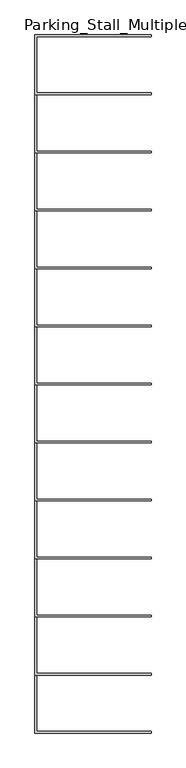
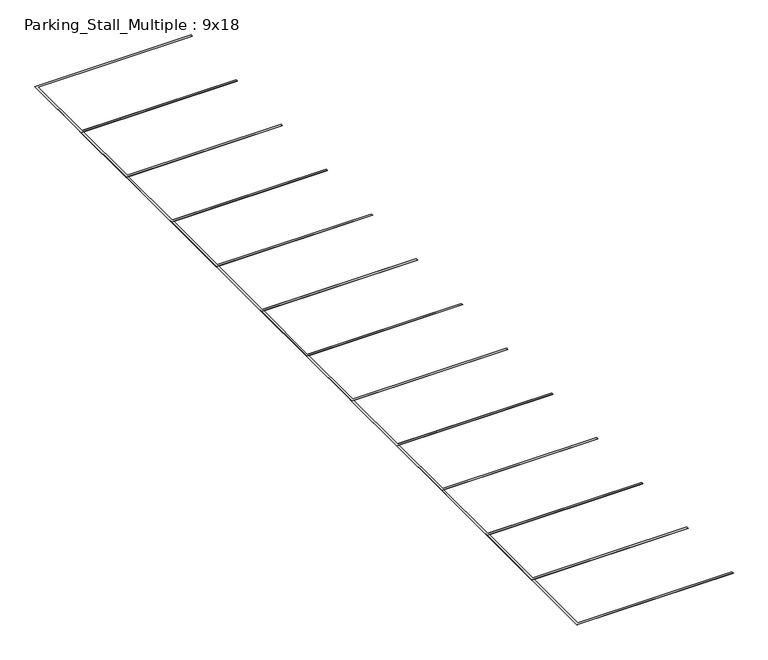
"""IFC4 building model written with IfcOpenShell, lengths in millimetres: proxy geometry, Parking_Stall_Multiple : 9x18."""

from ifc_helpers import new_model, si_unit, origin, origin_with_axes, place, context, project, spatial, polyline, outline, extrude, source, transform, mapped, element, save


def parking_stall_multiple_9x18_87ab82d0(model_context):
    return source(origin(), model_context, "Body", "SweptSolid", [
        extrude(outline(polyline([(5486.4, 30175.2), (0.0, 30175.2), (0.0, 32994.6), (5486.4, 32994.6), (5486.4, 32918.4), (76.2, 32918.4), (76.2, 30251.4), (5486.4, 30251.4), (5486.4, 30175.2)])), origin_with_axes(), (0.0, 0.0, 1.0), 6.35),
        extrude(outline(polyline([(5486.4, 27432.0), (0.0, 27432.0), (0.0, 30251.4), (5486.4, 30251.4), (5486.4, 30175.2), (76.2, 30175.2), (76.2, 27508.2), (5486.4, 27508.2), (5486.4, 27432.0)])), origin_with_axes(), (0.0, 0.0, 1.0), 6.35),
        extrude(outline(polyline([(5486.4, 24688.8), (0.0, 24688.8), (0.0, 27508.2), (5486.4, 27508.2), (5486.4, 27432.0), (76.2, 27432.0), (76.2, 24765.0), (5486.4, 24765.0), (5486.4, 24688.8)])), origin_with_axes(), (0.0, 0.0, 1.0), 6.35),
        extrude(outline(polyline([(5486.4, 21945.6), (0.0, 21945.6), (0.0, 24765.0), (5486.4, 24765.0), (5486.4, 24688.8), (76.2, 24688.8), (76.2, 22021.8), (5486.4, 22021.8), (5486.4, 21945.6)])), origin_with_axes(), (0.0, 0.0, 1.0), 6.35),
        extrude(outline(polyline([(5486.4, 19202.4), (0.0, 19202.4), (0.0, 22021.8), (5486.4, 22021.8), (5486.4, 21945.6), (76.2, 21945.6), (76.2, 19278.6), (5486.4, 19278.6), (5486.4, 19202.4)])), origin_with_axes(), (0.0, 0.0, 1.0), 6.35),
        extrude(outline(polyline([(5486.4, 16459.2), (0.0, 16459.2), (0.0, 19278.6), (5486.4, 19278.6), (5486.4, 19202.4), (76.2, 19202.4), (76.2, 16535.4), (5486.4, 16535.4), (5486.4, 16459.2)])), origin_with_axes(), (0.0, 0.0, 1.0), 6.35),
        extrude(outline(polyline([(5486.4, 13716.0), (0.0, 13716.0), (0.0, 16535.4), (5486.4, 16535.4), (5486.4, 16459.2), (76.2, 16459.2), (76.2, 13792.2), (5486.4, 13792.2), (5486.4, 13716.0)])), origin_with_axes(), (0.0, 0.0, 1.0), 6.35),
        extrude(outline(polyline([(5486.4, 10972.8), (0.0, 10972.8), (0.0, 13792.2), (5486.4, 13792.2), (5486.4, 13716.0), (76.2, 13716.0), (76.2, 11049.0), (5486.4, 11049.0), (5486.4, 10972.8)])), origin_with_axes(), (0.0, 0.0, 1.0), 6.35),
        extrude(outline(polyline([(5486.4, 8229.6), (0.0, 8229.6), (0.0, 11049.0), (5486.4, 11049.0), (5486.4, 10972.8), (76.2, 10972.8), (76.2, 8305.8), (5486.4, 8305.8), (5486.4, 8229.6)])), origin_with_axes(), (0.0, 0.0, 1.0), 6.35),
        extrude(outline(polyline([(5486.4, 5486.4), (0.0, 5486.4), (0.0, 8305.8), (5486.4, 8305.8), (5486.4, 8229.6), (76.2, 8229.6), (76.2, 5562.6), (5486.4, 5562.6), (5486.4, 5486.4)])), origin_with_axes(), (0.0, 0.0, 1.0), 6.35),
        extrude(outline(polyline([(5486.4, 2743.2), (0.0, 2743.2), (0.0, 5562.6), (5486.4, 5562.6), (5486.4, 5486.4), (76.2, 5486.4), (76.2, 2819.4), (5486.4, 2819.4), (5486.4, 2743.2)])), origin_with_axes(), (0.0, 0.0, 1.0), 6.35),
        extrude(outline(polyline([(5486.4, 0.0), (0.0, 0.0), (0.0, 2819.4), (5486.4, 2819.4), (5486.4, 2743.2), (76.2, 2743.2), (76.2, 76.2), (5486.4, 76.2), (5486.4, 0.0)])), origin_with_axes(), (0.0, 0.0, 1.0), 6.35),
    ])


if __name__ == "__main__":
    model = new_model("IFC4")
    model_context = context("Model", 3, world=origin())
    ifc_project = project(units=[si_unit("LENGTHUNIT", "METRE", prefix="MILLI")], contexts=[model_context])
    site = spatial("IfcSite", under=ifc_project)
    building = spatial("IfcBuilding", under=site)
    placement = place(None, origin())
    parking_stall_multiple_9x18_shape = parking_stall_multiple_9x18_87ab82d0(model_context)
    element("IfcBuildingElementProxy", 1, Name="Parking_Stall_Multiple : 9x18", ObjectType="Parking_Stall_Multiple : 9x18", at=placement, inside=building, context=model_context, shape_type="MappedRepresentation", body=[
        mapped(parking_stall_multiple_9x18_shape, transform((0.0, 0.0, 0.0), x_axis=(1.0, 0.0, 0.0), y_axis=(0.0, 1.0, 0.0), z_axis=(0.0, 0.0, 1.0))),
    ])
    save(model, "model.ifc")

# Revit data of these elements
# Type "Parking_Stall_Multiple : 9x18"
#   Type Mark = "PK-1"
#   Parking_Width_M = 9' - 0"
#   Parking_Run_Length [instance default] = 65' - 0"
#   Parking_Line_Width = 0' - 3"
#   Parking_Length_M = 18' - 0"
#   Single_Parking_Visibility [instance default] = no
#   Parking_ADA_Symbol = no
#   ParkingUnitsArray [instance default] = 7
#   ParkingUnits [instance default] = 7
#   Multiple_Parking_Visibility [instance default] = yes
#   Parking_Line_Material = none
# Element 1 (IfcBuildingElementProxy, "Parking_Stall_Multiple : 9x18")
#   Parking_Run_Length = 106' - 6.45777"
#   ParkingUnitsArray = 12
#   ParkingUnits = 12
